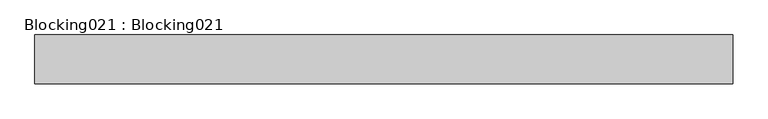
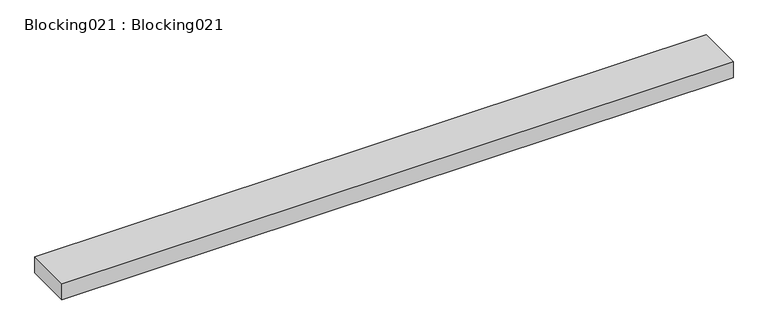
"""IFC4 building model written with IfcOpenShell, lengths in millimetres: proxy geometry, Blocking021 : Blocking021."""

from ifc_helpers import new_model, si_unit, frame, origin, place, context, project, spatial, polyline, outline, extrude, source, transform, mapped, element, save


def blocking021_blocking021_18cc6730(model_context):
    return source(origin(), model_context, "Body", "SweptSolid", [
        extrude(outline(polyline([(14383.0178845, -4497.8425368), (14383.0178845, -4637.5425368), (12383.0178845, -4637.5425368), (12383.0178845, -4497.8425368), (14383.0178845, -4497.8425368)])), frame((0.0, 0.0, 38360.096), z_axis=(0.0, 0.0, 1.0), x_axis=(1.0, 0.0, 0.0)), (0.0, 0.0, 1.0), 50.8),
    ])


if __name__ == "__main__":
    model = new_model("IFC4")
    model_context = context("Model", 3, world=origin())
    ifc_project = project(units=[si_unit("LENGTHUNIT", "METRE", prefix="MILLI")], contexts=[model_context])
    site = spatial("IfcSite", under=ifc_project)
    building = spatial("IfcBuilding", under=site)
    placement = place(None, origin())
    blocking021_blocking021_shape = blocking021_blocking021_18cc6730(model_context)
    element("IfcBuildingElementProxy", 1, Name="Blocking021 : Blocking021", ObjectType="Blocking021 : Blocking021", at=placement, inside=building, context=model_context, shape_type="MappedRepresentation", body=[
        mapped(blocking021_blocking021_shape, transform((0.0, 0.0, 0.0), x_axis=(1.0, 0.0, 0.0), y_axis=(0.0, 1.0, 0.0), z_axis=(0.0, 0.0, 1.0))),
    ])
    save(model, "model.ifc")

# Revit data of these elements
# Type "Blocking021 : Blocking021"
#   NameOverride = "Blocking021"
# Element 1 (IfcBuildingElementProxy, "Blocking021 : Blocking021")
#   Materials on its faces: "WOOD BLOCKING AS REQUIRED"
# Materials
#   "WOOD BLOCKING AS REQUIRED": class "Unassigned", colour RGB 166 124 85, transparency 0, Cost = 0
